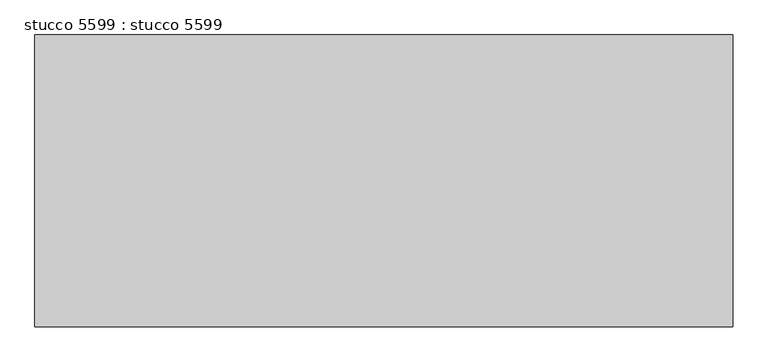
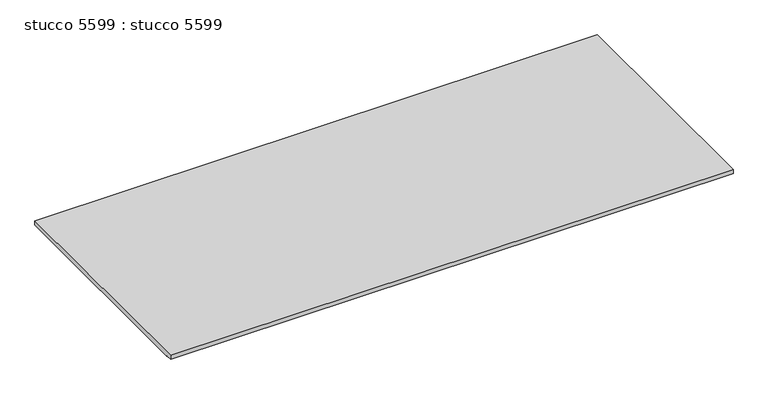
"""IFC4 building model written with IfcOpenShell, lengths in millimetres: proxy geometry, stucco 5599 : stucco 5599."""

from ifc_helpers import new_model, si_unit, frame, origin, place, context, project, spatial, polyline, outline, extrude, source, transform, mapped, element, save


def stucco_5599_stucco_5599_8cd41aec(model_context):
    return source(origin(), model_context, "Body", "SweptSolid", [
        extrude(outline(polyline([(-4690.5092773, 39712.8039618), (-5503.7598427, 39712.8039618), (-5503.7598427, 39714.0839618), (-5526.1930267, 39714.0839618), (-5526.1930267, 39728.9941181), (-4690.5092773, 39728.9941181), (-4690.5092773, 39712.8039618)])), frame((12383.0178845, 0.0, 0.0), z_axis=(1.0, 0.0, 0.0), x_axis=(0.0, 1.0, 0.0)), (0.0, 0.0, 1.0), 2000.0),
    ])


if __name__ == "__main__":
    model = new_model("IFC4")
    model_context = context("Model", 3, world=origin())
    ifc_project = project(units=[si_unit("LENGTHUNIT", "METRE", prefix="MILLI")], contexts=[model_context])
    site = spatial("IfcSite", under=ifc_project)
    building = spatial("IfcBuilding", under=site)
    placement = place(None, origin())
    stucco_5599_stucco_5599_shape = stucco_5599_stucco_5599_8cd41aec(model_context)
    element("IfcBuildingElementProxy", 1, Name="stucco 5599 : stucco 5599", ObjectType="stucco 5599 : stucco 5599", at=placement, inside=building, context=model_context, shape_type="MappedRepresentation", body=[
        mapped(stucco_5599_stucco_5599_shape, transform((0.0, 0.0, 0.0), x_axis=(1.0, 0.0, 0.0), y_axis=(0.0, 1.0, 0.0), z_axis=(0.0, 0.0, 1.0))),
    ])
    save(model, "model.ifc")

# Revit data of these elements
# Type "stucco 5599 : stucco 5599"
#   NameOverride = "stucco"
# Element 1 (IfcBuildingElementProxy, "stucco 5599 : stucco 5599")
#   Materials on its faces: "7/8\" SMOOTH TROWEL EXTERIOR STUCCO"
# Materials
#   "7/8\" SMOOTH TROWEL EXTERIOR STUCCO": class "Unassigned", colour RGB 255 255 255, transparency 0, Cost = 0
